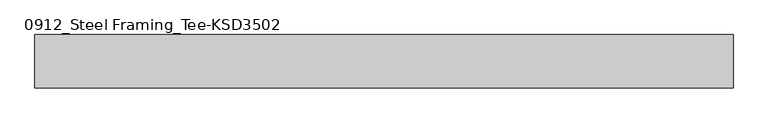
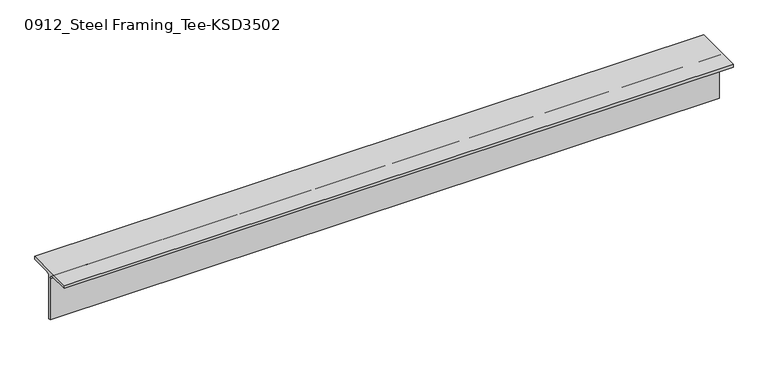
"""IFC4 building model written with IfcOpenShell, lengths in millimetres: member geometry, 0912_Steel Framing_Tee-KSD3502 : H_SB_ASB_CT-150x150x6.5x9."""

from ifc_helpers import new_model, si_unit, point, frame, frame_2d, origin, place, context, project, spatial, polyline, circle_curve, trimmed, segment, composite_curve, outline, extrude, source, transform, mapped, element, save


def member_0912_steel_framing_tee_ksd3502_fccfafc7(model_context):
    return source(origin(), model_context, "Body", "SweptSolid", [
        extrude(outline(composite_curve([segment(polyline([(-75.0, 75.0), (75.0, 75.0), (75.0, 66.0), (16.25, 66.0)]), True, "CONTINUOUS"), segment(trimmed(circle_curve(frame_2d((16.25, 53.0)), 13.0), [point((16.25, 66.0))], [point((3.25, 53.0))], True, "CARTESIAN"), True, "CONTINUOUS"), segment(polyline([(3.25, 53.0), (3.25, -75.0), (-3.25, -75.0), (-3.25, 53.0)]), True, "CONTINUOUS"), segment(trimmed(circle_curve(frame_2d((-16.25, 53.0)), 13.0), [point((-3.25, 53.0))], [point((-16.25, 66.0))], True, "CARTESIAN"), True, "CONTINUOUS"), segment(polyline([(-16.25, 66.0), (-75.0, 66.0), (-75.0, 75.0)]), True, "CONTINUOUS")], self_intersect=False)), frame((-983.95, 0.0, 0.0), z_axis=(1.0, 0.0, 0.0), x_axis=(0.0, 1.0, 0.0)), (0.0, 0.0, 1.0), 1967.9),
    ])


if __name__ == "__main__":
    model = new_model("IFC4")
    model_context = context("Model", 3, world=origin())
    ifc_project = project(units=[si_unit("LENGTHUNIT", "METRE", prefix="MILLI")], contexts=[model_context])
    site = spatial("IfcSite", under=ifc_project)
    building = spatial("IfcBuilding", under=site)
    placement = place(None, origin())
    member_0912_steel_framing_tee_ksd3502_shape = member_0912_steel_framing_tee_ksd3502_fccfafc7(model_context)
    element("IfcMember", 1, ObjectType="0912_Steel Framing_Tee-KSD3502 : H_SB_ASB_CT-150x150x6.5x9", at=placement, inside=building, context=model_context, shape_type="MappedRepresentation", body=[
        mapped(member_0912_steel_framing_tee_ksd3502_shape, transform((0.0, 0.0, 0.0), x_axis=(1.0, 0.0, 0.0), y_axis=(0.0, 1.0, 0.0), z_axis=(0.0, 0.0, 1.0))),
    ])
    save(model, "model.ifc")

# Revit data of these elements
# Type "0912_Steel Framing_Tee-KSD3502 : H_SB_ASB_CT-150x150x6.5x9"
#   H_WM Code_1 = "S01AA003-00001 | Main Steel Structure Fabrication Work | Shelter/Building | Light Steel - Standard (30KG/M>Weight) | Material: (   )"
#   H_WM Code_2 = "S03AA029-00001 | Main Steel Structure Erection Work | Shelter/Building | Light Steel (30KG/M>Weight) | Material: (   )"
#   H_WM Code_3 = "S01AA010-00001 | Main Steel Structure Fabrication Work | Shelter/Building | Steel Painting/Coating | for Non-Fireproofed Steel Surface, Surface Preparation, Primer, Second & Final Coat | Material: (   )"
#   H_Q'ty Cal Type Tag = "SB-Q2"
#   Width = 15.0 cm
#   Web Thickness = 0.65 cm
#   Web Fillet = 1.3 cm
#   Section Area = 23.39 cm²
#   Perimeter = 0.60 m²/m
#   Nominal Weight = 18.40 kgf/m
#   Height = 15.0 cm
#   Flange Thickness = 0.9 cm
#   Centroid Vertical = 7.5 cm
#   Centroid Horizontal = 7.5 cm
#   Length [instance default] = 1.5000 m
#   Structural Material [instance default] = Steel, 45-345
#   Warping Constant = (empty or 0)
#   Torsional Moment of Inertia = 0
#   Section Name Key = ""
#   Plastic Modulus weak axis = 0
#   Plastic Modulus strong axis = 0
#   Moment of Inertia weak axis = 0
#   Moment of Inertia strong axis = 0
#   Elastic Modulus weak axis = 0
#   Elastic Modulus strong axis = 0
#   Bolt Spacing = 0
#   Assembly Code = ""
# Element 1 (IfcMember, "0912_Steel Framing_Tee-KSD3502 : H_SB_ASB_CT-150x150x6.5x9")
#   Structural Material = none
# Materials
#   "Steel, 45-345": class "Metal", colour RGB 189 187 185, transparency 0, Description = "Steel 345 MPa", Cost = 0
